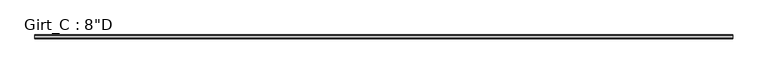
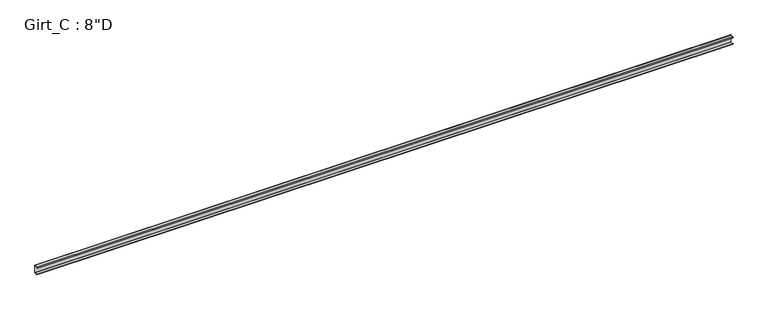
"""IFC4 building model written with IfcOpenShell, lengths in millimetres: beam geometry."""

from ifc_helpers import new_model, si_unit, point, frame, frame_2d, origin, place, context, project, spatial, polyline, circle_curve, trimmed, segment, composite_curve, outline, extrude, source, transform, mapped, element, save


def beam_f3872ff4(model_context):
    return source(origin(), model_context, "Body", "SweptSolid", [
        extrude(outline(composite_curve([segment(polyline([(-87.5109375, 101.6), (-3.3734375, 101.6)]), True, "CONTINUOUS"), segment(trimmed(circle_curve(frame_2d((-3.3734375, 96.8375)), 4.7625), [point((-3.3734375, 101.6))], [point((1.3890625, 96.8375))], False, "CARTESIAN"), True, "CONTINUOUS"), segment(polyline([(1.3890625, 96.8375), (1.3890625, -96.8375)]), True, "CONTINUOUS"), segment(trimmed(circle_curve(frame_2d((-3.3734375, -96.8375)), 4.7625), [point((1.3890625, -96.8375))], [point((-3.3734375, -101.6))], False, "CARTESIAN"), True, "CONTINUOUS"), segment(polyline([(-3.3734375, -101.6), (-87.5109375, -101.6), (-99.7792647, -86.979177), (-97.6510975, -85.1934327), (-86.2154765, -98.821875), (-3.2694106, -98.821875)]), True, "CONTINUOUS"), segment(trimmed(circle_curve(frame_2d((-3.3748024, -96.8389339)), 1.9857399), [point((-3.2694106, -98.821875))], [point((-1.3890625, -96.8389339))], True, "CARTESIAN"), True, "CONTINUOUS"), segment(polyline([(-1.3890625, -96.8389339), (-1.3890625, 96.8381931)]), True, "CONTINUOUS"), segment(trimmed(circle_curve(frame_2d((-3.3741066, 96.8381931)), 1.9850441), [point((-1.3890625, 96.8381931))], [point((-3.3005807, 98.821875))], True, "CARTESIAN"), True, "CONTINUOUS"), segment(polyline([(-3.3005807, 98.821875), (-86.2154765, 98.821875), (-97.6278742, 85.221109), (-99.7560415, 87.0068534), (-87.5109375, 101.6)]), True, "CONTINUOUS")], self_intersect=False)), frame((-9337.675, 0.0, 0.0), z_axis=(1.0, 0.0, 0.0), x_axis=(0.0, 1.0, 0.0)), (0.0, 0.0, 1.0), 18453.1),
    ])


if __name__ == "__main__":
    model = new_model("IFC4")
    model_context = context("Model", 3, world=origin())
    ifc_project = project(units=[si_unit("LENGTHUNIT", "METRE", prefix="MILLI")], contexts=[model_context])
    site = spatial("IfcSite", under=ifc_project)
    building = spatial("IfcBuilding", under=site)
    placement = place(None, origin())
    beam_shape = beam_f3872ff4(model_context)
    element("IfcBeam", 1, ObjectType="Girt_C : 8\"D", at=placement, inside=building, context=model_context, shape_type="MappedRepresentation", body=[
        mapped(beam_shape, transform((0.0, 0.0, 0.0), x_axis=(1.0, 0.0, 0.0), y_axis=(0.0, 1.0, 0.0), z_axis=(0.0, 0.0, 1.0))),
    ])
    save(model, "model.ifc")

# Revit data of these elements
# Type "Girt_C : 8\"D"
#   half leg = 0' - 1 3/4"
#   Web_Thickness = 0' - 0 7/64"
#   Length [instance default] = 10' - 0"
#   Leg_1 = 0' - 3 1/2"
#   Height = 0' - 8"
#   Structural Material [instance default] = none
# Element 1 (IfcBeam, "Girt_C : 8\"D")
#   Structural Material = CEE' SECTION (8.0x3.5C - SEE STRUCT. DWGS)
#   Materials on its faces: "CEE' SECTION (8.0x3.5C - SEE STRUCT. DWGS)"
# Materials
#   "CEE' SECTION (8.0x3.5C - SEE STRUCT. DWGS)": class "Metal", colour RGB 137 146 153, transparency 0, Description = "Steel, mill finish", Cost = 0
